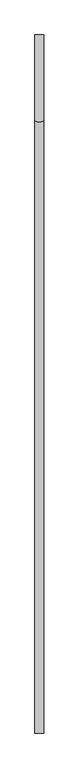
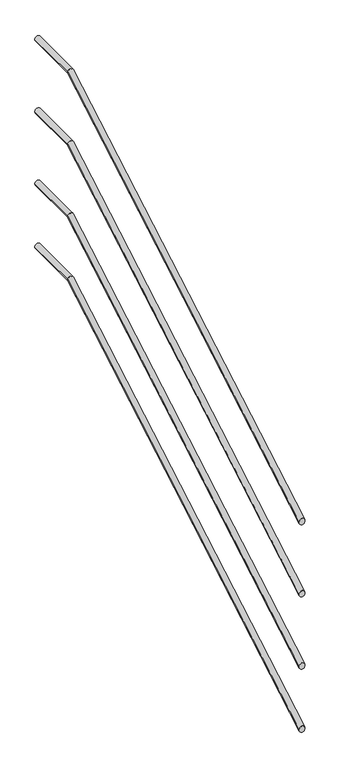
"""IFC4 building model written with IfcOpenShell, lengths in millimetres: railing geometry."""

from ifc_helpers import new_model, si_unit, frame, origin, place, context, project, spatial, circle_curve, ellipse_curve, source, transform, mapped, element, save
from ifc_brep_helpers import plane_surface, cylinder_surface, advanced_brep


def railing_a9f54978(model_context):
    return source(origin(), model_context, "Body", "AdvancedBrep", [
        advanced_brep(
        [(-3259.6, 13399.5208589, 4296.7361432), (-3289.6, 13399.5208589, 4296.7361432), (-3259.6, 15503.5584173, 5517.9030398), (-3289.6, 15503.5584173, 5517.9030398), (-3259.6, 15799.5208589, 5517.9030398), (-3289.6, 15799.5208589, 5517.9030398)],
        [
            (0, 1, ellipse_curve(frame((-3274.6, 13399.5208589, 4296.7361432), z_axis=(0.0, -1.0, 0.0), x_axis=(0.0, 0.0, -1.0)), 17.3433672, 15.0)),
            (1, 0, ellipse_curve(frame((-3274.6, 13399.5208589, 4296.7361432), z_axis=(0.0, -1.0, 0.0), x_axis=(0.0, 0.0, -1.0)), 17.3433672, 15.0)),
            (0, 2),
            (2, 3, ellipse_curve(frame((-3274.6, 15503.5584173, 5517.9030398), z_axis=(0.0, -0.9656303515230849, -0.2599192648062159), x_axis=(0.0, 0.2599192648062168, -0.9656303515230846)), 15.5338945, 15.0)),
            (3, 1),
            (3, 2, ellipse_curve(frame((-3274.6, 15503.5584173, 5517.9030398), z_axis=(0.0, -0.9656303515230849, -0.2599192648062159), x_axis=(0.0, 0.2599192648062168, -0.9656303515230846)), 15.5338945, 15.0)),
            (4, 5, circle_curve(frame((-3274.6, 15799.5208589, 5517.9030398), z_axis=(0.0, 1.0, 0.0), x_axis=(-1.0, 0.0, 0.0)), 15.0)),
            (5, 4, circle_curve(frame((-3274.6, 15799.5208589, 5517.9030398), z_axis=(0.0, 1.0, 0.0), x_axis=(-1.0, 0.0, 0.0)), 15.0)),
            (2, 4),
            (5, 3),
        ],
        [
            plane_surface(frame((-3274.6, 13399.5208589, 4314.0795104), z_axis=(0.0, -1.0, 0.0), x_axis=(0.0, 0.0, 1.0))),
            cylinder_surface(frame((-3274.6, 13407.0504368, 4301.1062512), z_axis=(0.0, -0.8648839515651925, -0.5019718620848959), x_axis=(-1.0, 0.0, 0.0)), 15.0),
            plane_surface(frame((-3274.6, 15799.5208589, 5532.9030398), z_axis=(0.0, 1.0, 0.0), x_axis=(0.0, 0.0, 1.0))),
            cylinder_surface(frame((-3274.6, 15499.5208589, 5517.9030398), z_axis=(0.0, -1.0, 0.0), x_axis=(-1.0, 0.0, 0.0)), 15.0),
        ],
        [
            (0, [[1, 2]]),
            (1, [[-1, 3, 4, 5]]),
            (1, [[-2, -5, 6, -3]]),
            (2, [[7, 8]]),
            (3, [[-4, 9, -8, 10]]),
            (3, [[-6, -10, -7, -9]]),
        ],
    ),
        advanced_brep(
        [(-3259.6, 13399.5208589, 3496.7361432), (-3289.6, 13399.5208589, 3496.7361432), (-3259.6, 15503.5584173, 4717.9030398), (-3289.6, 15503.5584173, 4717.9030398), (-3259.6, 15799.5208589, 4717.9030398), (-3289.6, 15799.5208589, 4717.9030398)],
        [
            (0, 1, ellipse_curve(frame((-3274.6, 13399.5208589, 3496.7361432), z_axis=(0.0, -1.0, 0.0), x_axis=(0.0, 0.0, -1.0)), 17.3433672, 15.0)),
            (1, 0, ellipse_curve(frame((-3274.6, 13399.5208589, 3496.7361432), z_axis=(0.0, -1.0, 0.0), x_axis=(0.0, 0.0, -1.0)), 17.3433672, 15.0)),
            (0, 2),
            (2, 3, ellipse_curve(frame((-3274.6, 15503.5584173, 4717.9030398), z_axis=(0.0, -0.9656303515230849, -0.2599192648062159), x_axis=(0.0, 0.2599192648062168, -0.9656303515230846)), 15.5338945, 15.0)),
            (3, 1),
            (3, 2, ellipse_curve(frame((-3274.6, 15503.5584173, 4717.9030398), z_axis=(0.0, -0.9656303515230849, -0.2599192648062159), x_axis=(0.0, 0.2599192648062168, -0.9656303515230846)), 15.5338945, 15.0)),
            (4, 5, circle_curve(frame((-3274.6, 15799.5208589, 4717.9030398), z_axis=(0.0, 1.0, 0.0), x_axis=(-1.0, 0.0, 0.0)), 15.0)),
            (5, 4, circle_curve(frame((-3274.6, 15799.5208589, 4717.9030398), z_axis=(0.0, 1.0, 0.0), x_axis=(-1.0, 0.0, 0.0)), 15.0)),
            (2, 4),
            (5, 3),
        ],
        [
            plane_surface(frame((-3274.6, 13399.5208589, 3514.0795104), z_axis=(0.0, -1.0, 0.0), x_axis=(0.0, 0.0, 1.0))),
            cylinder_surface(frame((-3274.6, 13407.0504368, 3501.1062512), z_axis=(0.0, -0.8648839515651925, -0.5019718620848959), x_axis=(-1.0, 0.0, 0.0)), 15.0),
            plane_surface(frame((-3274.6, 15799.5208589, 4732.9030398), z_axis=(0.0, 1.0, 0.0), x_axis=(0.0, 0.0, 1.0))),
            cylinder_surface(frame((-3274.6, 15499.5208589, 4717.9030398), z_axis=(0.0, -1.0, 0.0), x_axis=(-1.0, 0.0, 0.0)), 15.0),
        ],
        [
            (0, [[1, 2]]),
            (1, [[-1, 3, 4, 5]]),
            (1, [[-2, -5, 6, -3]]),
            (2, [[7, 8]]),
            (3, [[-4, 9, -8, 10]]),
            (3, [[-6, -10, -7, -9]]),
        ],
    ),
        advanced_brep(
        [(-3259.6, 13399.5208589, 3896.7361432), (-3289.6, 13399.5208589, 3896.7361432), (-3259.6, 15503.5584173, 5117.9030398), (-3289.6, 15503.5584173, 5117.9030398), (-3259.6, 15799.5208589, 5117.9030398), (-3289.6, 15799.5208589, 5117.9030398)],
        [
            (0, 1, ellipse_curve(frame((-3274.6, 13399.5208589, 3896.7361432), z_axis=(0.0, -1.0, 0.0), x_axis=(0.0, 0.0, -1.0)), 17.3433672, 15.0)),
            (1, 0, ellipse_curve(frame((-3274.6, 13399.5208589, 3896.7361432), z_axis=(0.0, -1.0, 0.0), x_axis=(0.0, 0.0, -1.0)), 17.3433672, 15.0)),
            (0, 2),
            (2, 3, ellipse_curve(frame((-3274.6, 15503.5584173, 5117.9030398), z_axis=(0.0, -0.9656303515230849, -0.2599192648062159), x_axis=(0.0, 0.2599192648062168, -0.9656303515230846)), 15.5338945, 15.0)),
            (3, 1),
            (3, 2, ellipse_curve(frame((-3274.6, 15503.5584173, 5117.9030398), z_axis=(0.0, -0.9656303515230849, -0.2599192648062159), x_axis=(0.0, 0.2599192648062168, -0.9656303515230846)), 15.5338945, 15.0)),
            (4, 5, circle_curve(frame((-3274.6, 15799.5208589, 5117.9030398), z_axis=(0.0, 1.0, 0.0), x_axis=(-1.0, 0.0, 0.0)), 15.0)),
            (5, 4, circle_curve(frame((-3274.6, 15799.5208589, 5117.9030398), z_axis=(0.0, 1.0, 0.0), x_axis=(-1.0, 0.0, 0.0)), 15.0)),
            (2, 4),
            (5, 3),
        ],
        [
            plane_surface(frame((-3274.6, 13399.5208589, 3914.0795104), z_axis=(0.0, -1.0, 0.0), x_axis=(0.0, 0.0, 1.0))),
            cylinder_surface(frame((-3274.6, 13407.0504368, 3901.1062512), z_axis=(0.0, -0.8648839515651925, -0.5019718620848959), x_axis=(-1.0, 0.0, 0.0)), 15.0),
            plane_surface(frame((-3274.6, 15799.5208589, 5132.9030398), z_axis=(0.0, 1.0, 0.0), x_axis=(0.0, 0.0, 1.0))),
            cylinder_surface(frame((-3274.6, 15499.5208589, 5117.9030398), z_axis=(0.0, -1.0, 0.0), x_axis=(-1.0, 0.0, 0.0)), 15.0),
        ],
        [
            (0, [[1, 2]]),
            (1, [[-1, 3, 4, 5]]),
            (1, [[-2, -5, 6, -3]]),
            (2, [[7, 8]]),
            (3, [[-4, 9, -8, 10]]),
            (3, [[-6, -10, -7, -9]]),
        ],
    ),
        advanced_brep(
        [(-3259.6, 13399.5208589, 3146.7361432), (-3289.6, 13399.5208589, 3146.7361432), (-3259.6, 15503.5584173, 4367.9030398), (-3289.6, 15503.5584173, 4367.9030398), (-3259.6, 15799.5208589, 4367.9030398), (-3289.6, 15799.5208589, 4367.9030398)],
        [
            (0, 1, ellipse_curve(frame((-3274.6, 13399.5208589, 3146.7361432), z_axis=(0.0, -1.0, 0.0), x_axis=(0.0, 0.0, -1.0)), 17.3433672, 15.0)),
            (1, 0, ellipse_curve(frame((-3274.6, 13399.5208589, 3146.7361432), z_axis=(0.0, -1.0, 0.0), x_axis=(0.0, 0.0, -1.0)), 17.3433672, 15.0)),
            (0, 2),
            (2, 3, ellipse_curve(frame((-3274.6, 15503.5584173, 4367.9030398), z_axis=(0.0, -0.9656303515230849, -0.2599192648062159), x_axis=(0.0, 0.2599192648062168, -0.9656303515230846)), 15.5338945, 15.0)),
            (3, 1),
            (3, 2, ellipse_curve(frame((-3274.6, 15503.5584173, 4367.9030398), z_axis=(0.0, -0.9656303515230849, -0.2599192648062159), x_axis=(0.0, 0.2599192648062168, -0.9656303515230846)), 15.5338945, 15.0)),
            (4, 5, circle_curve(frame((-3274.6, 15799.5208589, 4367.9030398), z_axis=(0.0, 1.0, 0.0), x_axis=(-1.0, 0.0, 0.0)), 15.0)),
            (5, 4, circle_curve(frame((-3274.6, 15799.5208589, 4367.9030398), z_axis=(0.0, 1.0, 0.0), x_axis=(-1.0, 0.0, 0.0)), 15.0)),
            (2, 4),
            (5, 3),
        ],
        [
            plane_surface(frame((-3274.6, 13399.5208589, 3164.0795104), z_axis=(0.0, -1.0, 0.0), x_axis=(0.0, 0.0, 1.0))),
            cylinder_surface(frame((-3274.6, 13407.0504368, 3151.1062512), z_axis=(0.0, -0.8648839515651925, -0.5019718620848959), x_axis=(-1.0, 0.0, 0.0)), 15.0),
            plane_surface(frame((-3274.6, 15799.5208589, 4382.9030398), z_axis=(0.0, 1.0, 0.0), x_axis=(0.0, 0.0, 1.0))),
            cylinder_surface(frame((-3274.6, 15499.5208589, 4367.9030398), z_axis=(0.0, -1.0, 0.0), x_axis=(-1.0, 0.0, 0.0)), 15.0),
        ],
        [
            (0, [[1, 2]]),
            (1, [[-1, 3, 4, 5]]),
            (1, [[-2, -5, 6, -3]]),
            (2, [[7, 8]]),
            (3, [[-4, 9, -8, 10]]),
            (3, [[-6, -10, -7, -9]]),
        ],
    ),
    ])


if __name__ == "__main__":
    model = new_model("IFC4")
    model_context = context("Model", 3, world=origin())
    ifc_project = project(units=[si_unit("LENGTHUNIT", "METRE", prefix="MILLI")], contexts=[model_context])
    site = spatial("IfcSite", under=ifc_project)
    building = spatial("IfcBuilding", under=site)
    placement = place(None, origin())
    railing_shape = railing_a9f54978(model_context)
    element("IfcRailing", 1, at=placement, inside=building, context=model_context, shape_type="MappedRepresentation", body=[
        mapped(railing_shape, transform((0.0, 0.0, 0.0), x_axis=(1.0, 0.0, 0.0), y_axis=(0.0, 1.0, 0.0), z_axis=(0.0, 0.0, 1.0))),
    ])
    save(model, "model.ifc")
